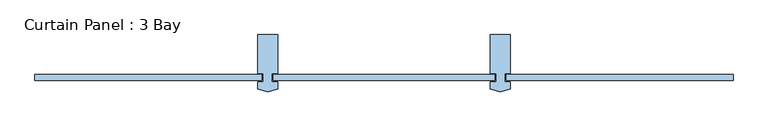
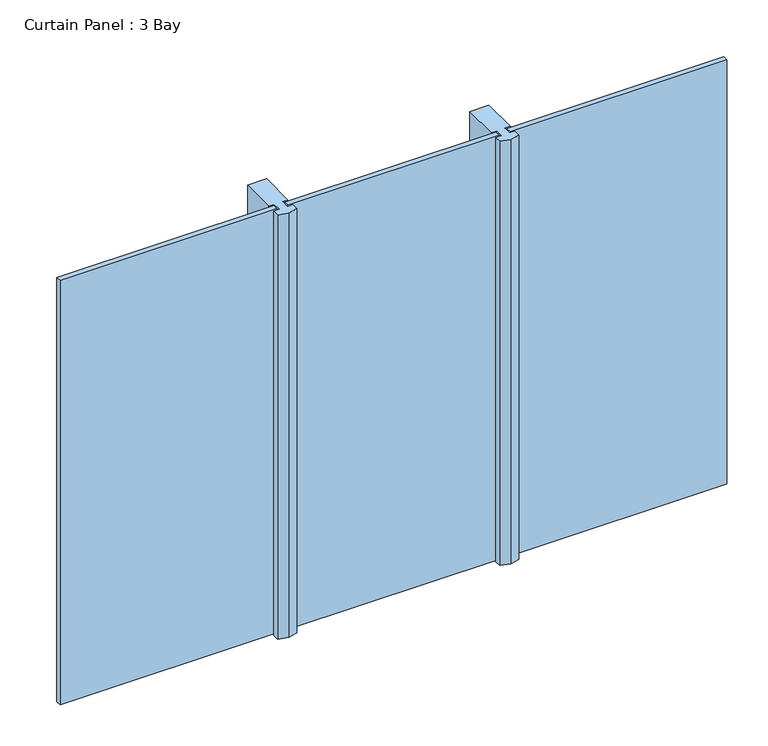
"""IFC4 building model written with IfcOpenShell, lengths in millimetres: window geometry, Curtain Panel : 3 Bay."""

from ifc_helpers import new_model, si_unit, origin, origin_with_axes, place, context, project, spatial, polyline, outline, extrude, source, transform, mapped, element, save


def curtain_panel_3_bay_7a2d2fe3(model_context):
    return source(origin(), model_context, "Body", "SweptSolid", [
        extrude(outline(polyline([(-472.0166667, -12.7), (-497.4166667, -12.7), (-497.4166667, -50.8), (-472.0166667, -50.8), (-472.0166667, -82.55), (-516.4666667, -95.25), (-560.9166667, -82.55), (-560.9166667, -50.8), (-535.5166667, -50.8), (-535.5166667, -12.7), (-560.9166667, -12.7), (-560.9166667, 158.75), (-472.0166667, 158.75), (-472.0166667, -12.7)])), origin_with_axes(), (0.0, 0.0, 1.0), 2086.1728929),
        extrude(outline(polyline([(472.0166667, -12.7), (472.0166667, 158.75), (560.9166667, 158.75), (560.9166667, -12.7), (535.5166667, -12.7), (535.5166667, -50.8), (560.9166667, -50.8), (560.9166667, -82.55), (516.4666667, -95.25), (472.0166667, -82.55), (472.0166667, -50.8), (497.4166667, -50.8), (497.4166667, -12.7), (472.0166667, -12.7)])), origin_with_axes(), (0.0, 0.0, 1.0), 2086.1728929),
        extrude(outline(polyline([(-491.0666667, -44.45), (-491.0666667, -19.05), (491.0666667, -19.05), (491.0666667, -44.45), (-491.0666667, -44.45)])), origin_with_axes(), (0.0, 0.0, 1.0), 2086.1728929),
        extrude(outline(polyline([(-1549.4, -44.45), (-1549.4, -19.05), (-541.8666667, -19.05), (-541.8666667, -44.45), (-1549.4, -44.45)])), origin_with_axes(), (0.0, 0.0, 1.0), 2086.1728929),
        extrude(outline(polyline([(541.8666667, -44.45), (541.8666667, -19.05), (1549.4, -19.05), (1549.4, -44.45), (541.8666667, -44.45)])), origin_with_axes(), (0.0, 0.0, 1.0), 2086.1728929),
    ])


if __name__ == "__main__":
    model = new_model("IFC4")
    model_context = context("Model", 3, world=origin())
    ifc_project = project(units=[si_unit("LENGTHUNIT", "METRE", prefix="MILLI")], contexts=[model_context])
    site = spatial("IfcSite", under=ifc_project)
    building = spatial("IfcBuilding", under=site)
    placement = place(None, origin())
    curtain_panel_3_bay_shape = curtain_panel_3_bay_7a2d2fe3(model_context)
    element("IfcWindow", 1, ObjectType="Curtain Panel : 3 Bay", at=placement, inside=building, context=model_context, shape_type="MappedRepresentation", body=[
        mapped(curtain_panel_3_bay_shape, transform((0.0, 0.0, 0.0), x_axis=(1.0, 0.0, 0.0), y_axis=(0.0, 1.0, 0.0), z_axis=(0.0, 0.0, 1.0))),
    ])
    save(model, "model.ifc")

# Revit data of these elements
# Type "Curtain Panel : 3 Bay"
#   Type Mark = "24"
#   Description = "The Aubin Academy Master Series"
#   Offset = 0' - 1 1/4"
# Element 1 (IfcWindow, "Curtain Panel : 3 Bay")
#   Materials on its faces: "Metal - Aluminum", "Glass"
# Materials
#   "Metal - Aluminum": class "Metal", colour RGB 247 247 247, transparency 0
#   "Glass": class "Glass", colour RGB 0 128 192, transparency 0.75, Description = "Soda Lime Glass", Cost = 0
